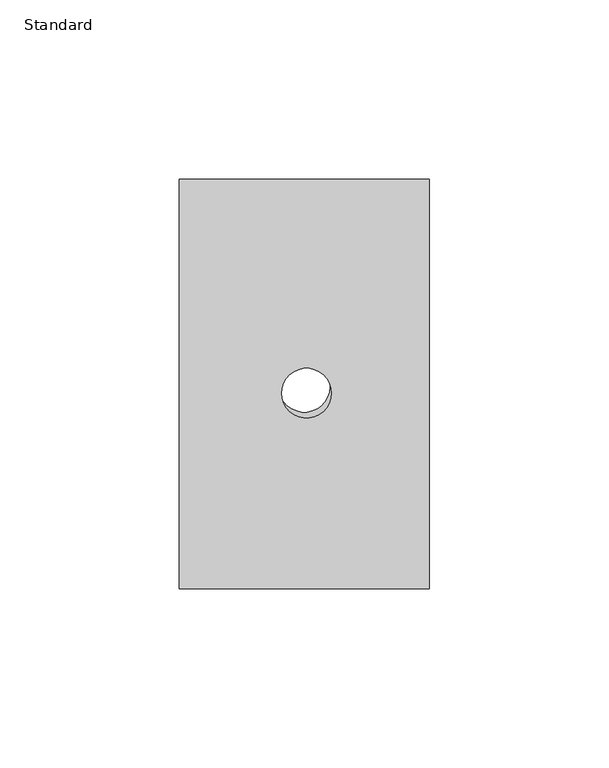
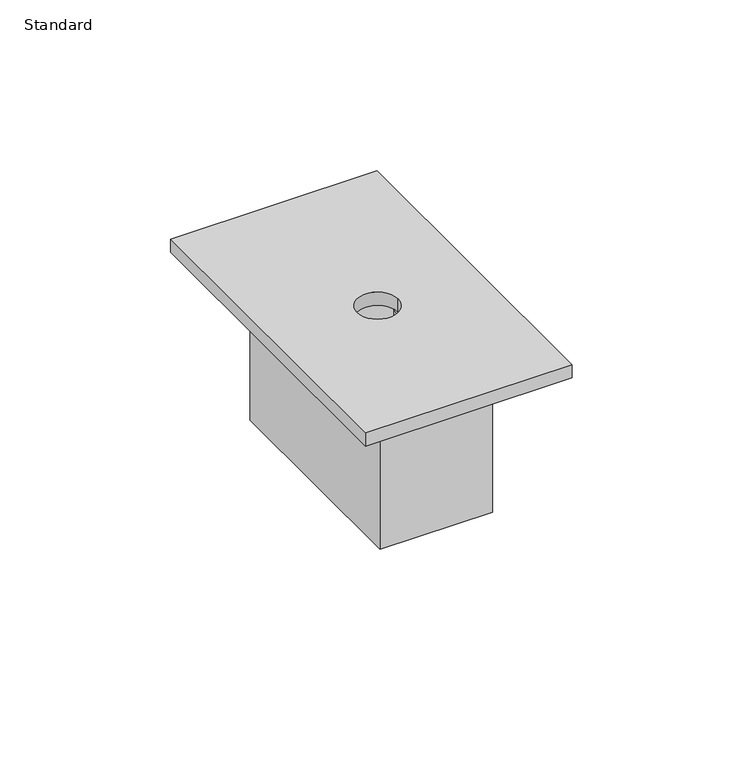
"""IFC4 building model written with IfcOpenShell, lengths in millimetres: proxy geometry, M_Receptacle -TV /Satellite Socket : Standard."""

from ifc_helpers import new_model, si_unit, point, frame, frame_2d, origin, origin_with_axes, place, context, project, spatial, polyline, circle_curve, trimmed, segment, composite_curve, outline, extrude, source, transform, mapped, element, save


def standard_8138c307(model_context):
    return source(origin(), model_context, "Body", "SweptSolid", [
        extrude(outline(polyline([(34.925, 57.15), (34.925, -57.15), (-34.925, -57.15), (-34.925, 57.15), (34.925, 57.15)]), holes=[composite_curve([segment(trimmed(circle_curve(frame_2d((0.6039572, -2.5749254)), 6.9441889), [point((-6.3402317, -2.5749254))], [point((7.5481461, -2.5749254))], True, "CARTESIAN"), True, "CONTINUOUS"), segment(trimmed(circle_curve(frame_2d((0.6039572, -2.5749254)), 6.9441889), [point((7.5481461, -2.5749254))], [point((-6.3402317, -2.5749254))], True, "CARTESIAN"), True, "CONTINUOUS")], self_intersect=False)]), origin_with_axes(), (0.0, 0.0, 1.0), 4.7625),
        extrude(outline(polyline([(19.05, 38.1), (19.05, -38.1), (-19.05, -38.1), (-19.05, 38.1), (19.05, 38.1)]), holes=[composite_curve([segment(trimmed(circle_curve(frame_2d((0.0, -0.79375)), 7.0675853), [point((-7.0675853, -0.79375))], [point((7.0675853, -0.79375))], True, "CARTESIAN"), True, "CONTINUOUS"), segment(trimmed(circle_curve(frame_2d((0.0, -0.79375)), 7.0675853), [point((7.0675853, -0.79375))], [point((-7.0675853, -0.79375))], True, "CARTESIAN"), True, "CONTINUOUS")], self_intersect=False)]), frame((0.0, 0.0, -53.975), z_axis=(0.0, 0.0, 1.0), x_axis=(1.0, 0.0, 0.0)), (0.0, 0.0, 1.0), 53.975),
    ])


if __name__ == "__main__":
    model = new_model("IFC4")
    model_context = context("Model", 3, world=origin())
    ifc_project = project(units=[si_unit("LENGTHUNIT", "METRE", prefix="MILLI")], contexts=[model_context])
    site = spatial("IfcSite", under=ifc_project)
    building = spatial("IfcBuilding", under=site)
    placement = place(None, origin())
    standard_shape = standard_8138c307(model_context)
    element("IfcBuildingElementProxy", 1, Name="M_Receptacle -TV /Satellite Socket : Standard", ObjectType="M_Receptacle -TV /Satellite Socket : Standard", at=placement, inside=building, context=model_context, shape_type="MappedRepresentation", body=[
        mapped(standard_shape, transform((0.0, 0.0, 0.0), x_axis=(1.0, 0.0, 0.0), y_axis=(0.0, 1.0, 0.0), z_axis=(0.0, 0.0, 1.0))),
    ])
    save(model, "model.ifc")

# Revit data of these elements
# Type "M_Receptacle -TV /Satellite Socket : Standard"
#   Type Mark = "M_Receptacle -TV"
#   Classification.OmniClass.21.Number = "21-04 50 30 50"
#   Classification.MasterFormat.Description = "Wiring Devices"
#   Classification.OmniClass.22.Number = "22-26 27 26"
#   Classification.OmniClass.21.Description = "Wiring Devices"
#   Classification.UniFormat.II.Description = "Wiring Devices"
#   Classification.MasterFormat.Number = "26 27 26"
#   Classification.OmniClass.23.Number = "23-35 27 11"
#   Classification.OmniClass.22.Description = "Wiring Devices"
#   Classification.OmniClass.23.Description = "Electrical Receptacles"
#   Classification.UniFormat.II.Number = "D5030.50"
#   COBie.Type.CreatedBy = "info@mma.ie"
#   COBie.Type.CreatedOn = "2017-07-25T10:15:16"
#   COBie.Type.Name = "M_Receptacle -TV"
#   COBie.Type.Category = "23-35 27 11 : Electrical Receptacles"
#   COBie.Type.Description = "M_Receptacle -TV /Satellite Socket_Standard"
#   COBie.Type.AssetType = "Fixed"
#   COBie.Type.Manufacturer = ""
#   COBie.Type.ModelNumber = ""
#   Keynote = "26 27 26.A"
#   COBie.Type.ReplacementCost = 0
#   Switch Voltage = 220 V
#   Recep.Width = 69.85 mm
#   Recep.Load = 180 VA
#   Recep.Height = 114.3 mm
#   Load = 180 VA
#   Default Elevation = 460 mm
#   COBie.Type = yes
#   Recep.Material = Stainless Steel
#   Load Classification = Receptacle
#   Assembly Code = ""
# Materials
#   "Stainless Steel": class "Metal", colour RGB 120 120 120, transparency 0, Description = "Stainless Steel 18/8", Cost = 0
